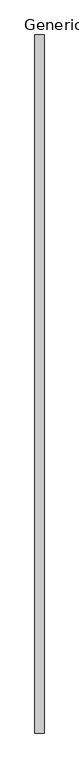
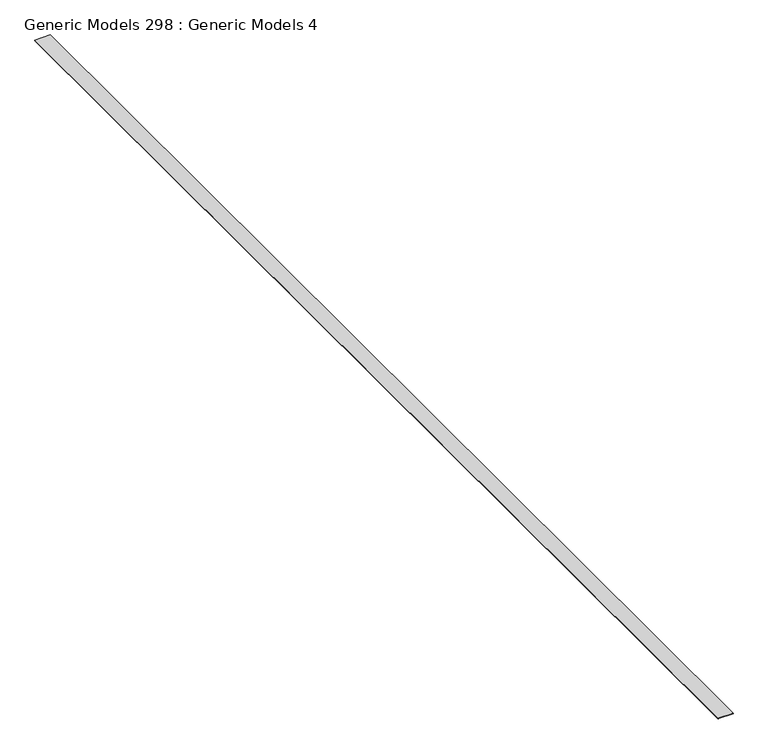
"""IFC4 building model written with IfcOpenShell, lengths in millimetres: proxy geometry, Generic Models 298 : Generic Models 4."""

from ifc_helpers import new_model, si_unit, frame, origin, place, context, project, spatial, polyline, outline, extrude, source, transform, mapped, element, save


def generic_models_298_generic_models_4_47bf6a21(model_context):
    return source(origin(), model_context, "Body", "SweptSolid", [
        extrude(outline(polyline([(87307.251867, 24984.1772257), (87410.4113509, 24984.1772257), (87410.4113509, 17097.4772257), (87307.251867, 17097.4772257), (87307.251867, 24984.1772257)])), frame((0.0, 0.0, 124904.8777896), z_axis=(0.0, 0.0, 1.0), x_axis=(1.0, 0.0, 0.0)), (0.0, 0.0, 1.0), 1.3753749),
        extrude(outline(polyline([(87307.251867, 24984.1772257), (87410.4113509, 24984.1772257), (87410.4113509, 17097.4772257), (87307.251867, 17097.4772257), (87307.251867, 24984.1772257)])), frame((0.0, 0.0, 124908.2714479), z_axis=(0.0, 0.0, 1.0), x_axis=(1.0, 0.0, 0.0)), (0.0, 0.0, 1.0), 1.3753749),
    ])


if __name__ == "__main__":
    model = new_model("IFC4")
    model_context = context("Model", 3, world=origin())
    ifc_project = project(units=[si_unit("LENGTHUNIT", "METRE", prefix="MILLI")], contexts=[model_context])
    site = spatial("IfcSite", under=ifc_project)
    building = spatial("IfcBuilding", under=site)
    placement = place(None, origin())
    generic_models_298_generic_models_4_shape = generic_models_298_generic_models_4_47bf6a21(model_context)
    element("IfcBuildingElementProxy", 1, Name="Generic Models 298 : Generic Models 4", ObjectType="Generic Models 298 : Generic Models 4", at=placement, inside=building, context=model_context, shape_type="MappedRepresentation", body=[
        mapped(generic_models_298_generic_models_4_shape, transform((0.0, 0.0, 0.0), x_axis=(1.0, 0.0, 0.0), y_axis=(0.0, 1.0, 0.0), z_axis=(0.0, 0.0, 1.0))),
    ])
    save(model, "model.ifc")

# Revit data of these elements
# Element 1 (IfcBuildingElementProxy, "Generic Models 298 : Generic Models 4")
#   Materials on its faces: "_BED OF SEALANT (ABOVE/BELOW FLASHING)"
# Materials
#   "_BED OF SEALANT (ABOVE/BELOW FLASHING)": class "Generic", colour RGB 253 192 103, transparency 0, Cost = 0
